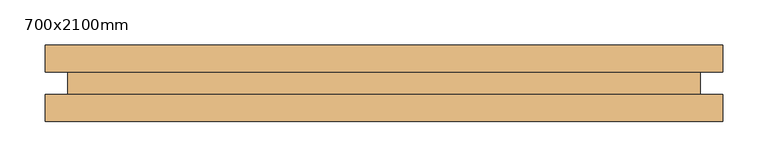
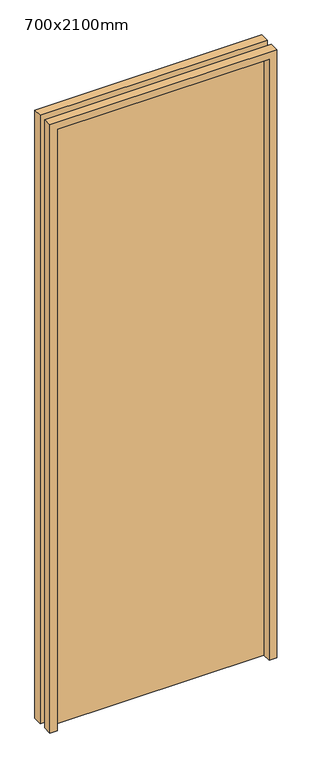
"""IFC4 building model written with IfcOpenShell, lengths in millimetres: door geometry, WWm-SingleSolid-Flush : 700x2100mm."""

from ifc_helpers import new_model, si_unit, frame, origin, origin_with_axes, place, context, project, spatial, polyline, outline, extrude, source, transform, mapped, element, save


def door_700x2100mm_84725625(model_context):
    return source(origin(), model_context, "Body", "SweptSolid", [
        extrude(outline(polyline([(2125.0, -375.0), (0.0, -375.0), (0.0, -350.0), (2100.0, -350.0), (2100.0, 350.0), (0.0, 350.0), (0.0, 375.0), (2125.0, 375.0), (2125.0, -375.0)])), frame((0.0, -42.5, 0.0), z_axis=(0.0, 1.0, 0.0), x_axis=(0.0, 0.0, 1.0)), (0.0, 0.0, 1.0), 30.0),
        extrude(outline(polyline([(2125.0, 375.0), (2125.0, -375.0), (0.0, -375.0), (0.0, -350.0), (2100.0, -350.0), (2100.0, 350.0), (0.0, 350.0), (0.0, 375.0), (2125.0, 375.0)])), frame((0.0, 12.5, 0.0), z_axis=(0.0, 1.0, 0.0), x_axis=(0.0, 0.0, 1.0)), (0.0, 0.0, 1.0), 30.0),
        extrude(outline(polyline([(350.0, 37.5), (350.0, -12.5), (-350.0, -12.5), (-350.0, 37.5), (350.0, 37.5)])), origin_with_axes(), (0.0, 0.0, 1.0), 2100.0),
    ])


if __name__ == "__main__":
    model = new_model("IFC4")
    model_context = context("Model", 3, world=origin())
    ifc_project = project(units=[si_unit("LENGTHUNIT", "METRE", prefix="MILLI")], contexts=[model_context])
    site = spatial("IfcSite", under=ifc_project)
    building = spatial("IfcBuilding", under=site)
    placement = place(None, origin())
    door_700x2100mm_shape = door_700x2100mm_84725625(model_context)
    element("IfcDoor", 1, ObjectType="WWm-SingleSolid-Flush : 700x2100mm", at=placement, inside=building, context=model_context, shape_type="MappedRepresentation", body=[
        mapped(door_700x2100mm_shape, transform((0.0, 0.0, 0.0), x_axis=(1.0, 0.0, 0.0), y_axis=(0.0, 1.0, 0.0), z_axis=(0.0, 0.0, 1.0))),
    ])
    save(model, "model.ifc")

# Revit data of these elements
# Type "WWm-SingleSolid-Flush : 700x2100mm"
#   Type Mark = "EX1-53"
#   Construction Type Id = "MDOOR"
#   Assembly Code = "C1020"
#   Analytic Construction = "Metal"
#   Thickness = 50 mm
#   Thermal Resistance (R) = 0.270117 (m²·K)/W
#   Heat Transfer Coefficient (U) = 3.7021 W/(m²·K)
#   Height = 2100 mm
#   Trim Projection Ext = 30 mm
#   Trim Projection Int = 30 mm
#   Trim Width = 25 mm
#   Width = 700 mm
#   Not 90 Degree [instance default] = no
#   90 Degree [instance default] = yes
#   Door Material = WW-EC-RGB-White
#   Frame Material = WW-EC-RGB-White
#   Visual Light Transmittance = 0
#   Solar Heat Gain Coefficient = 0
#   Function = (empty or 0)
#   Wall Closure = (empty or 0)
# Element 1 (IfcDoor, "WWm-SingleSolid-Flush : 700x2100mm")
#   Materials on its faces: "WW-EC-RGB-White"
# Materials
#   "WW-EC-RGB-White": class "Generic", colour RGB 255 255 255, transparency 0, Comments = "If region requests off-white, swith asset color to RGB 231-228-220", Description = "Generic Color", Cost = 0
